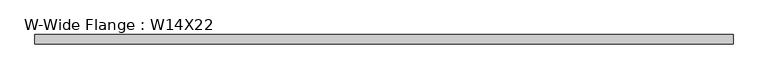
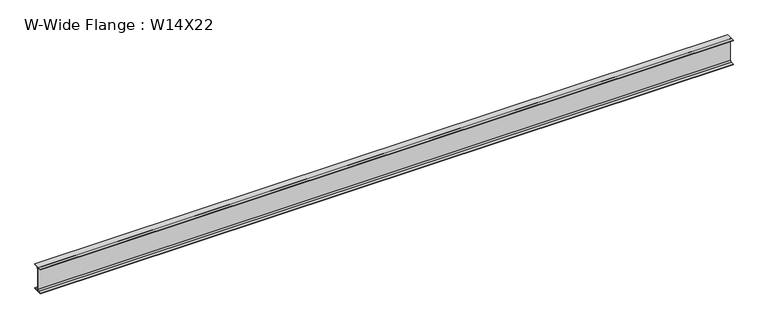
"""IFC4 building model written with IfcOpenShell, lengths in millimetres: beam geometry, W-Wide Flange : W14X22."""

from ifc_helpers import new_model, si_unit, point, frame, frame_2d, origin, place, context, project, spatial, polyline, circle_curve, trimmed, segment, composite_curve, outline, extrude, source, transform, mapped, element, save


def w_wide_flange_w14x22_2e51511a(model_context):
    return source(origin(), model_context, "Body", "SweptSolid", [
        extrude(outline(composite_curve([segment(polyline([(63.5, -165.481), (63.5, -173.99), (-63.5, -173.99), (-63.5, -165.481), (-21.3995, -165.481)]), True, "CONTINUOUS"), segment(trimmed(circle_curve(frame_2d((-21.3995, -147.0025)), 18.4785), [point((-21.3995, -165.481))], [point((-2.921, -147.0025))], True, "CARTESIAN"), True, "CONTINUOUS"), segment(polyline([(-2.921, -147.0025), (-2.921, 147.0025)]), True, "CONTINUOUS"), segment(trimmed(circle_curve(frame_2d((-21.3995, 147.0025)), 18.4785), [point((-2.921, 147.0025))], [point((-21.3995, 165.481))], True, "CARTESIAN"), True, "CONTINUOUS"), segment(polyline([(-21.3995, 165.481), (-63.5, 165.481), (-63.5, 173.99), (63.5, 173.99), (63.5, 165.481), (21.3995, 165.481)]), True, "CONTINUOUS"), segment(trimmed(circle_curve(frame_2d((21.3995, 147.0025)), 18.4785), [point((21.3995, 165.481))], [point((2.921, 147.0025))], True, "CARTESIAN"), True, "CONTINUOUS"), segment(polyline([(2.921, 147.0025), (2.921, -147.0025)]), True, "CONTINUOUS"), segment(trimmed(circle_curve(frame_2d((21.3995, -147.0025)), 18.4785), [point((2.921, -147.0025))], [point((21.3995, -165.481))], True, "CARTESIAN"), True, "CONTINUOUS"), segment(polyline([(21.3995, -165.481), (63.5, -165.481)]), True, "CONTINUOUS")], self_intersect=False)), frame((-4672.838, 0.0, 0.0), z_axis=(1.0, 0.0, 0.0), x_axis=(0.0, 1.0, 0.0)), (0.0, 0.0, 1.0), 9340.088),
    ])


if __name__ == "__main__":
    model = new_model("IFC4")
    model_context = context("Model", 3, world=origin())
    ifc_project = project(units=[si_unit("LENGTHUNIT", "METRE", prefix="MILLI")], contexts=[model_context])
    site = spatial("IfcSite", under=ifc_project)
    building = spatial("IfcBuilding", under=site)
    placement = place(None, origin())
    w_wide_flange_w14x22_shape = w_wide_flange_w14x22_2e51511a(model_context)
    element("IfcBeam", 1, ObjectType="W-Wide Flange : W14X22", at=placement, inside=building, context=model_context, shape_type="MappedRepresentation", body=[
        mapped(w_wide_flange_w14x22_shape, transform((0.0, 0.0, 0.0), x_axis=(1.0, 0.0, 0.0), y_axis=(0.0, 1.0, 0.0), z_axis=(0.0, 0.0, 1.0))),
    ])
    save(model, "model.ifc")

# Revit data of these elements
# Type "W-Wide Flange : W14X22"
#   Assembly Code = "B10"
#   W = 22
#   Length [instance default] = 1524 mm
#   bf = 127 mm
#   d = 347.98 mm
#   k = 26.988 mm
#   k2 = 18.479 mm
#   tf = 8.509 mm
#   tw = 5.842 mm
#   A = 0.00418709 m²
#   Structural Material [instance default] = Steel ASTM A992
# Element 1 (IfcBeam, "W-Wide Flange : W14X22")
#   Structural Material = Aluminum, Anodized Red
#   Materials on its faces: "Aluminum, Anodized Red"
# Materials
#   "Steel ASTM A992": class "Metal", colour RGB 128 0 0, transparency 0, Description = "Structural steel 50ksi", Cost = 0
#   "Aluminum, Anodized Red": class "Metal", colour RGB 120 120 120, transparency 0, Description = "Anodized aluminum, red", Cost = 0
